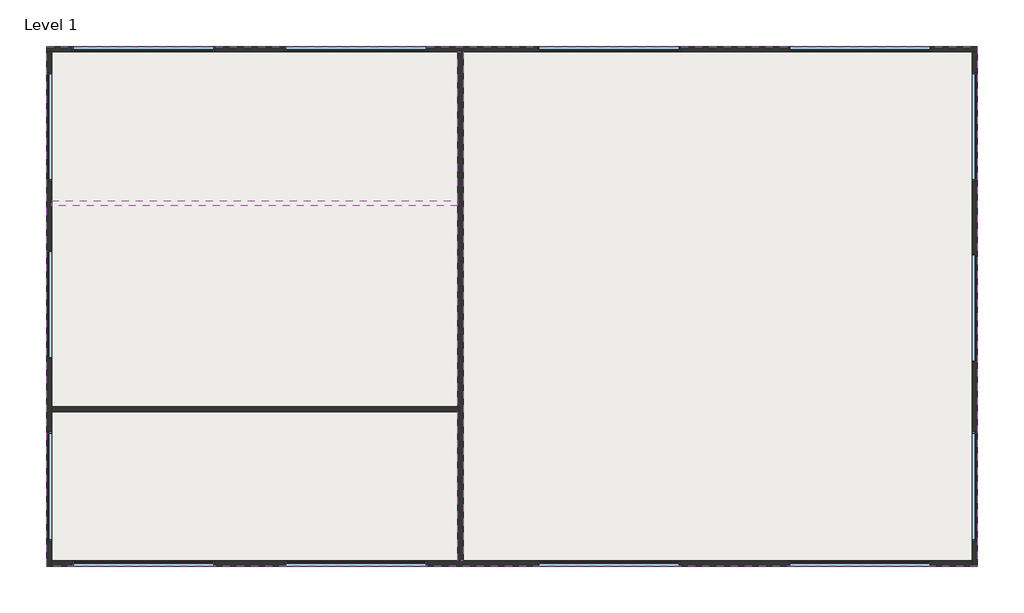
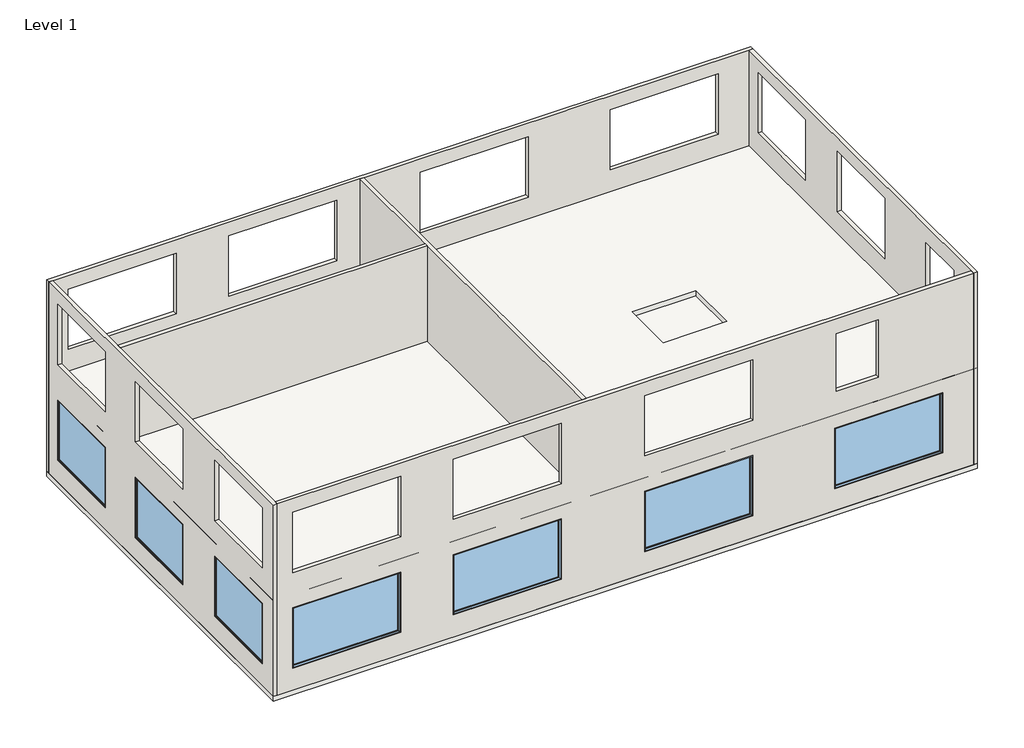
# One storey: 14 windows, 8 walls, 2 slabs.
"""IFC4 building model written with IfcOpenShell, lengths in millimetres."""

import ifcopenshell
import ifcopenshell.guid

model = None  # the IFC model being written
_history = None  # IfcOwnerHistory: only IFC2X3 demands one
_inside = {}  # id of a spatial element -> (the spatial element, [elements in it])
_under = {}  # id of a project, library or spatial element -> (it, [spatial elements below it])
_declared = {}  # id of a project -> (the project, [libraries it declares])
_typed = {}  # id of a type object -> (the type object, [elements of that type])
_made_of = {}  # id of a material, layer set ... -> (it, [elements and type objects made of it])


def new_model(schema):
    """Start an empty IFC model of exactly this schema.

    Asked for "IFC4X3", IfcOpenShell would pick the latest addendum, in which some entities
    have other attributes; the version numbers below select the first issue.
    IFC2X3 requires an IfcOwnerHistory on every rooted entity: one is made here for all.
    """
    global model, _history
    if schema == "IFC4X3":
        model = ifcopenshell.file(schema_version=(4, 3, 0, 0))
    else:
        model = ifcopenshell.file(schema=schema)
    _inside.clear()
    _under.clear()
    _declared.clear()
    _typed.clear()
    _made_of.clear()
    _history = None
    if model.schema == "IFC2X3":
        org = make("IfcOrganization", Name="unknown")
        user = make(
            "IfcPersonAndOrganization",
            ThePerson=make("IfcPerson", FamilyName="unknown"),
            TheOrganization=org,
        )
        app = make(
            "IfcApplication",
            ApplicationDeveloper=org,
            Version="unknown",
            ApplicationFullName="unknown",
            ApplicationIdentifier="unknown",
        )
        _history = make(
            "IfcOwnerHistory",
            OwningUser=user,
            OwningApplication=app,
            ChangeAction="ADDED",
            CreationDate=0,
        )
    return model


def make(cls, **values):
    """One entity of the class cls with the attributes given. An attribute that is None is left unset."""
    return model.create_entity(
        cls, **{name: value for name, value in values.items() if value is not None}
    )


def rooted(cls, **values):
    """An entity with a GlobalId (a new one), such as an element, a storey or a relation."""
    return make(cls, GlobalId=ifcopenshell.guid.new(), OwnerHistory=_history, **values)


def si_unit(unit_type, name, prefix=None):
    """IfcSIUnit, for example si_unit("LENGTHUNIT", "METRE", prefix="MILLI")."""
    return make("IfcSIUnit", UnitType=unit_type, Prefix=prefix, Name=name)


def assignment(units):
    """IfcUnitAssignment: the units of a project."""
    return None if units is None else make("IfcUnitAssignment", Units=units)


def point(xyz):
    """IfcCartesianPoint."""
    return None if xyz is None else make("IfcCartesianPoint", Coordinates=xyz)


def direction(xyz):
    """IfcDirection."""
    return None if xyz is None else make("IfcDirection", DirectionRatios=xyz)


def frame(location, z_axis=None, x_axis=None):
    """IfcAxis2Placement3D, a coordinate frame: its origin and axes. An axis left out is left unset."""
    return make(
        "IfcAxis2Placement3D",
        Location=point(location),
        Axis=direction(z_axis),
        RefDirection=direction(x_axis),
    )


def origin():
    """The frame at (0, 0, 0) with its axes left unset."""
    return frame((0.0, 0.0, 0.0))


def origin_with_axes():
    """The frame at (0, 0, 0) with the z axis (0, 0, 1) and the x axis (1, 0, 0) written out."""
    return frame((0.0, 0.0, 0.0), z_axis=(0.0, 0.0, 1.0), x_axis=(1.0, 0.0, 0.0))


def place(relative_to, where):
    """IfcLocalPlacement: puts the frame where relative to a parent placement (None: the world)."""
    return make(
        "IfcLocalPlacement", PlacementRelTo=relative_to, RelativePlacement=where
    )


def context(
    kind, dimensions, precision=None, world=None, true_north=None, identifier=None
):
    """IfcGeometricRepresentationContext, for example the 3D "Model" context."""
    return make(
        "IfcGeometricRepresentationContext",
        ContextIdentifier=identifier,
        ContextType=kind,
        CoordinateSpaceDimension=dimensions,
        Precision=precision,
        WorldCoordinateSystem=world,
        TrueNorth=true_north,
    )


def project(units=None, contexts=None):
    """IfcProject with its units and contexts."""
    return rooted(
        "IfcProject",
        Name="project",
        RepresentationContexts=contexts,
        UnitsInContext=assignment(units),
    )


def spatial(cls, under=None, at=None, **own):
    """A site, building, storey or space (cls), placed at a placement, below another one or the project."""
    s = rooted(cls, ObjectPlacement=at, **own)
    if under is not None:
        _under.setdefault(under.id(), (under, []))[1].append(s)
    return s


def polyline(points):
    """IfcPolyline through the points."""
    return make("IfcPolyline", Points=[point(p) for p in points])


def outline(outer, holes=None, kind="AREA"):
    """IfcArbitraryClosedProfileDef: a profile drawn as a closed curve; with holes, ...WithVoids."""
    if holes is None:
        return make("IfcArbitraryClosedProfileDef", ProfileType=kind, OuterCurve=outer)
    return make(
        "IfcArbitraryProfileDefWithVoids",
        ProfileType=kind,
        OuterCurve=outer,
        InnerCurves=holes,
    )


def extrude(swept, where, along, depth):
    """IfcExtrudedAreaSolid: the profile swept, set in the frame where, extruded along a direction by depth."""
    return make(
        "IfcExtrudedAreaSolid",
        SweptArea=swept,
        Position=where,
        ExtrudedDirection=direction(along),
        Depth=depth,
    )


def faces_of(points, faces, orient=None, outer=None):
    """IfcFace entities. A face is a list of loops; a loop is a list of indices into points, from 0.

    orient and outer hold one flag for each loop. By default every Orientation is true, the
    first loop of a face is its IfcFaceOuterBound and the others are IfcFaceBound.
    """
    made = []
    for i, loops in enumerate(faces):
        bounds = []
        for j, loop in enumerate(loops):
            is_outer = j == 0 if outer is None else outer[i][j]
            bounds.append(
                make(
                    "IfcFaceOuterBound" if is_outer else "IfcFaceBound",
                    Bound=make("IfcPolyLoop", Polygon=[points[k] for k in loop]),
                    Orientation=True if orient is None else orient[i][j],
                )
            )
        made.append(make("IfcFace", Bounds=bounds))
    return made


def faceted_brep(points, faces, orient=None, outer=None, voids=None):
    """IfcFacetedBrep: a solid bounded by flat faces; with voids (closed shells), ...WithVoids."""
    shared = [point(p) for p in points]
    hull = make("IfcClosedShell", CfsFaces=faces_of(shared, faces, orient, outer))
    if voids is None:
        return make("IfcFacetedBrep", Outer=hull)
    return make(
        "IfcFacetedBrepWithVoids",
        Outer=hull,
        Voids=[
            make(cls, CfsFaces=faces_of(shared, fs, o, b)) for cls, fs, o, b in voids
        ],
    )


def shape(context_of_items, identifier, shape_type, items):
    """IfcShapeRepresentation: the items that make up one representation, for example the "Body"."""
    return make(
        "IfcShapeRepresentation",
        ContextOfItems=context_of_items,
        RepresentationIdentifier=identifier,
        RepresentationType=shape_type,
        Items=items,
    )


def source(mapping_origin, context_of_items, identifier, shape_type, items):
    """IfcRepresentationMap: a shape defined once, which mapped items show again and again."""
    return make(
        "IfcRepresentationMap",
        MappingOrigin=mapping_origin,
        MappedRepresentation=shape(context_of_items, identifier, shape_type, items),
    )


def transform(
    local_origin,
    x_axis=None,
    y_axis=None,
    z_axis=None,
    scale=None,
    scale2=None,
    scale3=None,
    uniform=True,
):
    """IfcCartesianTransformationOperator3D, or its non-uniform kind. x_axis, y_axis, z_axis: its Axis1, 2, 3."""
    if uniform:
        return make(
            "IfcCartesianTransformationOperator3D",
            Axis1=direction(x_axis),
            Axis2=direction(y_axis),
            LocalOrigin=point(local_origin),
            Scale=scale,
            Axis3=direction(z_axis),
        )
    return make(
        "IfcCartesianTransformationOperator3DnonUniform",
        Axis1=direction(x_axis),
        Axis2=direction(y_axis),
        LocalOrigin=point(local_origin),
        Scale=scale,
        Axis3=direction(z_axis),
        Scale2=scale2,
        Scale3=scale3,
    )


def mapped(mapping_source, mapping_target):
    """IfcMappedItem: shows the shape of a source again, moved by a transform."""
    return make(
        "IfcMappedItem", MappingSource=mapping_source, MappingTarget=mapping_target
    )


def made_of(thing, what):
    """Note that an element or type object is made of a material, layer set ...; save() writes the relation."""
    if what is not None:
        _made_of.setdefault(what.id(), (what, []))[1].append(thing)
    return thing


def element(
    cls,
    number,
    at=None,
    inside=None,
    cuts=None,
    type_object=None,
    material=None,
    context=None,
    identifier="Body",
    shape_type=None,
    held_by="IfcProductDefinitionShape",
    body=None,
    shapes=None,
    **own,
):
    """One element of the class cls, such as IfcWall. Its Tag is "e" and its number.

    at: its placement. inside: the storey or other place that contains it. cuts: it is an
    opening in that element (IfcRelVoidsElement). A single representation is given by context,
    identifier, shape_type and body (its items); several are given by shapes. held_by: the class
    of the entity that holds the representations. save() writes the other relations.
    """
    e = rooted(cls, Tag="e%d" % number, ObjectPlacement=at, **own)
    if body is not None:
        shapes = [shape(context, identifier, shape_type, body)]
    if shapes is not None:
        e.Representation = make(held_by, Representations=shapes)
    if inside is not None:
        _inside.setdefault(inside.id(), (inside, []))[1].append(e)
    if cuts is not None:
        rooted(
            "IfcRelVoidsElement", RelatingBuildingElement=cuts, RelatedOpeningElement=e
        )
    if type_object is not None:
        _typed.setdefault(type_object.id(), (type_object, []))[1].append(e)
    return made_of(e, material)


def aggregate(whole, parts):
    """IfcRelAggregates: a whole, such as a stair, and the parts it consists of."""
    return rooted("IfcRelAggregates", RelatingObject=whole, RelatedObjects=parts)


def save(model, path):
    """Write the relations noted so far, then the file.

    IfcRelAggregates (storeys below a building ...), IfcRelContainedInSpatialStructure (elements
    in a storey), IfcRelDefinesByType, IfcRelAssociatesMaterial and IfcRelDeclares: one each for
    every whole, place, type object, material and project.
    """
    for whole, parts in _under.values():
        aggregate(whole, parts)
    for where, things in _inside.values():
        rooted(
            "IfcRelContainedInSpatialStructure",
            RelatedElements=things,
            RelatingStructure=where,
        )
    for kind, things in _typed.values():
        rooted("IfcRelDefinesByType", RelatedObjects=things, RelatingType=kind)
    for what, things in _made_of.values():
        rooted("IfcRelAssociatesMaterial", RelatedObjects=things, RelatingMaterial=what)
    for by, libraries in _declared.values():
        rooted("IfcRelDeclares", RelatingContext=by, RelatedDefinitions=libraries)
    model.write(path)


def m_fixed_2500x_4228mm_fd5e51e7(model_context):
    return source(origin(), model_context, "Body", "SweptSolid", [
        extrude(outline(polyline([(-2050.8, 54.2), (2050.8, 54.2), (2050.8, 42.2), (-2050.8, 42.2), (-2050.8, 54.2)])), frame((0.0, 0.0, 368.0), z_axis=(0.0, 0.0, 1.0), x_axis=(1.0, 0.0, 0.0)), (0.0, 0.0, 1.0), 2374.0),
        extrude(outline(polyline([(2786.0, -2094.8), (324.0, -2094.8), (324.0, 2094.8), (2786.0, 2094.8), (2786.0, -2094.8)]), holes=[polyline([(2742.0, -2050.8), (2742.0, 2050.8), (368.0, 2050.8), (368.0, -2050.8), (2742.0, -2050.8)])]), frame((0.0, 26.2, 0.0), z_axis=(0.0, 1.0, 0.0), x_axis=(0.0, 0.0, 1.0)), (0.0, 0.0, 1.0), 44.0),
        extrude(outline(polyline([(2805.0, -2113.8), (305.0, -2113.8), (305.0, 2113.8), (2805.0, 2113.8), (2805.0, -2113.8)]), holes=[polyline([(2786.0, -2094.8), (2786.0, 2094.8), (324.0, 2094.8), (324.0, -2094.8), (2786.0, -2094.8)])]), frame((0.0, 26.2, 0.0), z_axis=(0.0, 1.0, 0.0), x_axis=(0.0, 0.0, 1.0)), (0.0, 0.0, 1.0), 63.0),
        extrude(outline(polyline([(2805.0, -2113.8), (305.0, -2113.8), (305.0, 2113.8), (2805.0, 2113.8), (2805.0, -2113.8)]), holes=[polyline([(2773.0, -2081.8), (2773.0, 2081.8), (337.0, 2081.8), (337.0, -2081.8), (2773.0, -2081.8)])]), frame((0.0, -63.2, 0.0), z_axis=(0.0, 1.0, 0.0), x_axis=(0.0, 0.0, 1.0)), (0.0, 0.0, 1.0), 89.4),
    ])


def m_fixed_2500x_4228mm_f14c179f(model_context):
    return source(origin(), model_context, "Body", "SweptSolid", [
        extrude(outline(polyline([(-2050.8, -54.2), (-2050.8, -42.2), (2050.8, -42.2), (2050.8, -54.2), (-2050.8, -54.2)])), frame((0.0, 0.0, 368.0), z_axis=(0.0, 0.0, 1.0), x_axis=(1.0, 0.0, 0.0)), (0.0, 0.0, 1.0), 2374.0),
        extrude(outline(polyline([(2786.0, -2094.8), (324.0, -2094.8), (324.0, 2094.8), (2786.0, 2094.8), (2786.0, -2094.8)]), holes=[polyline([(2742.0, -2050.8), (2742.0, 2050.8), (368.0, 2050.8), (368.0, -2050.8), (2742.0, -2050.8)])]), frame((0.0, -70.2, 0.0), z_axis=(0.0, 1.0, 0.0), x_axis=(0.0, 0.0, 1.0)), (0.0, 0.0, 1.0), 44.0),
        extrude(outline(polyline([(2805.0, -2113.8), (305.0, -2113.8), (305.0, 2113.8), (2805.0, 2113.8), (2805.0, -2113.8)]), holes=[polyline([(2786.0, -2094.8), (2786.0, 2094.8), (324.0, 2094.8), (324.0, -2094.8), (2786.0, -2094.8)])]), frame((0.0, -89.2, 0.0), z_axis=(0.0, 1.0, 0.0), x_axis=(0.0, 0.0, 1.0)), (0.0, 0.0, 1.0), 63.0),
        extrude(outline(polyline([(2805.0, -2113.8), (305.0, -2113.8), (305.0, 2113.8), (2805.0, 2113.8), (2805.0, -2113.8)]), holes=[polyline([(2773.0, -2081.8), (2773.0, 2081.8), (337.0, 2081.8), (337.0, -2081.8), (2773.0, -2081.8)])]), frame((0.0, -26.2, 0.0), z_axis=(0.0, 1.0, 0.0), x_axis=(0.0, 0.0, 1.0)), (0.0, 0.0, 1.0), 89.4),
    ])


def m_fixed_2500x_3220mm_df94f4d0(model_context):
    return source(origin(), model_context, "Body", "SweptSolid", [
        extrude(outline(polyline([(-1546.8, 54.2), (1546.8, 54.2), (1546.8, 42.2), (-1546.8, 42.2), (-1546.8, 54.2)])), frame((0.0, 0.0, 368.0), z_axis=(0.0, 0.0, 1.0), x_axis=(1.0, 0.0, 0.0)), (0.0, 0.0, 1.0), 2374.0),
        extrude(outline(polyline([(2786.0, -1590.8), (324.0, -1590.8), (324.0, 1590.8), (2786.0, 1590.8), (2786.0, -1590.8)]), holes=[polyline([(2742.0, -1546.8), (2742.0, 1546.8), (368.0, 1546.8), (368.0, -1546.8), (2742.0, -1546.8)])]), frame((0.0, 26.2, 0.0), z_axis=(0.0, 1.0, 0.0), x_axis=(0.0, 0.0, 1.0)), (0.0, 0.0, 1.0), 44.0),
        extrude(outline(polyline([(2805.0, -1609.8), (305.0, -1609.8), (305.0, 1609.8), (2805.0, 1609.8), (2805.0, -1609.8)]), holes=[polyline([(2786.0, -1590.8), (2786.0, 1590.8), (324.0, 1590.8), (324.0, -1590.8), (2786.0, -1590.8)])]), frame((0.0, 26.2, 0.0), z_axis=(0.0, 1.0, 0.0), x_axis=(0.0, 0.0, 1.0)), (0.0, 0.0, 1.0), 63.0),
        extrude(outline(polyline([(2805.0, -1609.8), (305.0, -1609.8), (305.0, 1609.8), (2805.0, 1609.8), (2805.0, -1609.8)]), holes=[polyline([(2773.0, -1577.8), (2773.0, 1577.8), (337.0, 1577.8), (337.0, -1577.8), (2773.0, -1577.8)])]), frame((0.0, -63.2, 0.0), z_axis=(0.0, 1.0, 0.0), x_axis=(0.0, 0.0, 1.0)), (0.0, 0.0, 1.0), 89.4),
    ])


def m_fixed_2500x_3220mm_8b997f8c(model_context):
    return source(origin(), model_context, "Body", "SweptSolid", [
        extrude(outline(polyline([(-1546.8, -54.2), (-1546.8, -42.2), (1546.8, -42.2), (1546.8, -54.2), (-1546.8, -54.2)])), frame((0.0, 0.0, 368.0), z_axis=(0.0, 0.0, 1.0), x_axis=(1.0, 0.0, 0.0)), (0.0, 0.0, 1.0), 2374.0),
        extrude(outline(polyline([(2786.0, -1590.8), (324.0, -1590.8), (324.0, 1590.8), (2786.0, 1590.8), (2786.0, -1590.8)]), holes=[polyline([(2742.0, -1546.8), (2742.0, 1546.8), (368.0, 1546.8), (368.0, -1546.8), (2742.0, -1546.8)])]), frame((0.0, -70.2, 0.0), z_axis=(0.0, 1.0, 0.0), x_axis=(0.0, 0.0, 1.0)), (0.0, 0.0, 1.0), 44.0),
        extrude(outline(polyline([(2805.0, -1609.8), (305.0, -1609.8), (305.0, 1609.8), (2805.0, 1609.8), (2805.0, -1609.8)]), holes=[polyline([(2786.0, -1590.8), (2786.0, 1590.8), (324.0, 1590.8), (324.0, -1590.8), (2786.0, -1590.8)])]), frame((0.0, -89.2, 0.0), z_axis=(0.0, 1.0, 0.0), x_axis=(0.0, 0.0, 1.0)), (0.0, 0.0, 1.0), 63.0),
        extrude(outline(polyline([(2805.0, -1609.8), (305.0, -1609.8), (305.0, 1609.8), (2805.0, 1609.8), (2805.0, -1609.8)]), holes=[polyline([(2773.0, -1577.8), (2773.0, 1577.8), (337.0, 1577.8), (337.0, -1577.8), (2773.0, -1577.8)])]), frame((0.0, -26.2, 0.0), z_axis=(0.0, 1.0, 0.0), x_axis=(0.0, 0.0, 1.0)), (0.0, 0.0, 1.0), 89.4),
    ])


model = new_model("IFC4")

# Units and contexts
model_context = context("Model", 3, world=origin())
ifc_project = project(units=[si_unit("LENGTHUNIT", "METRE", prefix="MILLI")], contexts=[model_context])

# Site, building, storey
site = spatial("IfcSite", under=ifc_project)
building = spatial("IfcBuilding", under=site)
storey = spatial("IfcBuildingStorey", under=building, Name="Level 1", Elevation=0.0)

# Slabs
placement = place(None, origin())
element("IfcSlab", 1, ObjectType="160mm Concrete With 50mm Metal Deck", at=placement, inside=storey, context=model_context, shape_type="Brep", body=[
    faceted_brep([(29068.464681, 11296.9802217, -210.0), (29068.464681, -4095.4197783, -210.0), (1484.064681, -4095.4197783, -210.0), (1484.064681, 11296.9802217, -210.0), (29068.464681, 11296.9802217, 0.0), (1484.064681, 11296.9802217, 0.0), (1484.064681, 11144.5802217, 0.0), (1484.064681, -4095.4197783, 0.0), (28916.064681, -4095.4197783, 0.0), (29068.464681, -4095.4197783, 0.0), (29068.464681, 11144.5802217, 0.0)], [[[0, 1, 2, 3]], [[4, 5, 6, 7, 8, 9, 10]], [[1, 0, 4, 10, 9]], [[2, 1, 9, 8, 7]], [[3, 2, 7, 6, 5]], [[0, 3, 5, 4]]]),
])
element("IfcSlab", 2, ObjectType="160mm Concrete With 50mm Metal Deck", at=placement, inside=storey, context=model_context, shape_type="SweptSolid", body=[
    extrude(outline(polyline([(29068.464681, 11296.9802217), (29068.464681, -4095.4197783), (1484.064681, -4095.4197783), (1484.064681, 11296.9802217), (29068.464681, 11296.9802217)]), holes=[polyline([(23070.5967133, 4620.1802217), (20570.5967133, 4620.1802217), (20570.5967133, 2520.1802217), (23070.5967133, 2520.1802217), (23070.5967133, 4620.1802217)])]), frame((0.0, 0.0, 3752.4), z_axis=(0.0, 0.0, 1.0), x_axis=(1.0, 0.0, 0.0)), (0.0, 0.0, 1.0), 210.0),
])

# Walls
element("IfcWall", 3, ObjectType="Generic - 152.4mm", at=placement, inside=storey, context=model_context, shape_type="Brep", body=[
    faceted_brep([(1484.064681, 11144.5802217, 0.0), (1636.464681, 11144.5802217, 0.0), (13676.064681, 11144.5802217, 0.0), (13828.464681, 11144.5802217, 0.0), (28916.064681, 11144.5802217, 0.0), (29068.464681, 11144.5802217, 0.0), (29068.464681, 11144.5802217, 7924.8), (28916.064681, 11144.5802217, 7924.8), (23222.9967133, 11144.5802217, 7924.8), (23070.5967133, 11144.5802217, 7924.8), (20570.5967133, 11144.5802217, 7924.8), (20418.1967133, 11144.5802217, 7924.8), (13828.464681, 11144.5802217, 7924.8), (13676.064681, 11144.5802217, 7924.8), (1636.464681, 11144.5802217, 7924.8), (1484.064681, 11144.5802217, 7924.8), (6474.064681, 11144.5802217, 902.4), (2246.464681, 11144.5802217, 902.4), (2246.464681, 11144.5802217, 3402.4), (6474.064681, 11144.5802217, 3402.4), (12766.064681, 11144.5802217, 902.4), (8538.464681, 11144.5802217, 902.4), (8538.464681, 11144.5802217, 3402.4), (12766.064681, 11144.5802217, 3402.4), (20266.064681, 11144.5802217, 902.4), (16038.464681, 11144.5802217, 902.4), (16038.464681, 11144.5802217, 3402.4), (20266.064681, 11144.5802217, 3402.4), (27706.064681, 11144.5802217, 902.4), (23478.464681, 11144.5802217, 902.4), (23478.464681, 11144.5802217, 3402.4), (27706.064681, 11144.5802217, 3402.4), (27706.064681, 11144.5802217, 4862.4), (23478.464681, 11144.5802217, 4862.4), (23478.464681, 11144.5802217, 7362.4), (27706.064681, 11144.5802217, 7362.4), (20266.064681, 11144.5802217, 4862.4), (16038.464681, 11144.5802217, 4862.4), (16038.464681, 11144.5802217, 7362.4), (20266.064681, 11144.5802217, 7362.4), (12766.064681, 11144.5802217, 4862.4), (8538.464681, 11144.5802217, 4862.4), (8538.464681, 11144.5802217, 7362.4), (12766.064681, 11144.5802217, 7362.4), (6474.064681, 11144.5802217, 4862.4), (2246.464681, 11144.5802217, 4862.4), (2246.464681, 11144.5802217, 7362.4), (6474.064681, 11144.5802217, 7362.4), (1484.064681, 11296.9802217, 0.0), (1484.064681, 11296.9802217, 7924.8), (29068.464681, 11296.9802217, 7924.8), (29068.464681, 11296.9802217, 0.0), (6474.064681, 11296.9802217, 902.4), (6474.064681, 11296.9802217, 3402.4), (2246.464681, 11296.9802217, 3402.4), (2246.464681, 11296.9802217, 902.4), (12766.064681, 11296.9802217, 902.4), (12766.064681, 11296.9802217, 3402.4), (8538.464681, 11296.9802217, 3402.4), (8538.464681, 11296.9802217, 902.4), (20266.064681, 11296.9802217, 902.4), (20266.064681, 11296.9802217, 3402.4), (16038.464681, 11296.9802217, 3402.4), (16038.464681, 11296.9802217, 902.4), (27706.064681, 11296.9802217, 902.4), (27706.064681, 11296.9802217, 3402.4), (23478.464681, 11296.9802217, 3402.4), (23478.464681, 11296.9802217, 902.4), (27706.064681, 11296.9802217, 4862.4), (27706.064681, 11296.9802217, 7362.4), (23478.464681, 11296.9802217, 7362.4), (23478.464681, 11296.9802217, 4862.4), (20266.064681, 11296.9802217, 4862.4), (20266.064681, 11296.9802217, 7362.4), (16038.464681, 11296.9802217, 7362.4), (16038.464681, 11296.9802217, 4862.4), (12766.064681, 11296.9802217, 4862.4), (12766.064681, 11296.9802217, 7362.4), (8538.464681, 11296.9802217, 7362.4), (8538.464681, 11296.9802217, 4862.4), (6474.064681, 11296.9802217, 4862.4), (6474.064681, 11296.9802217, 7362.4), (2246.464681, 11296.9802217, 7362.4), (2246.464681, 11296.9802217, 4862.4)], [[[0, 1, 2, 3, 4, 5, 6, 7, 8, 9, 10, 11, 12, 13, 14, 15], [16, 17, 18, 19], [20, 21, 22, 23], [24, 25, 26, 27], [28, 29, 30, 31], [32, 33, 34, 35], [36, 37, 38, 39], [40, 41, 42, 43], [44, 45, 46, 47]], [[48, 49, 50, 51], [52, 53, 54, 55], [56, 57, 58, 59], [60, 61, 62, 63], [64, 65, 66, 67], [68, 69, 70, 71], [72, 73, 74, 75], [76, 77, 78, 79], [80, 81, 82, 83]], [[5, 4, 3, 2, 1, 0, 48, 51]], [[15, 14, 13, 12, 11, 10, 9, 8, 7, 6, 50, 49]], [[6, 5, 51, 50]], [[0, 15, 49, 48]], [[53, 52, 16, 19]], [[54, 53, 19, 18]], [[55, 54, 18, 17]], [[52, 55, 17, 16]], [[57, 56, 20, 23]], [[58, 57, 23, 22]], [[59, 58, 22, 21]], [[56, 59, 21, 20]], [[61, 60, 24, 27]], [[62, 61, 27, 26]], [[63, 62, 26, 25]], [[60, 63, 25, 24]], [[65, 64, 28, 31]], [[66, 65, 31, 30]], [[67, 66, 30, 29]], [[64, 67, 29, 28]], [[69, 68, 32, 35]], [[70, 69, 35, 34]], [[71, 70, 34, 33]], [[68, 71, 33, 32]], [[73, 72, 36, 39]], [[74, 73, 39, 38]], [[75, 74, 38, 37]], [[72, 75, 37, 36]], [[77, 76, 40, 43]], [[78, 77, 43, 42]], [[79, 78, 42, 41]], [[76, 79, 41, 40]], [[81, 80, 44, 47]], [[82, 81, 47, 46]], [[83, 82, 46, 45]], [[80, 83, 45, 44]]]),
])
element("IfcWall", 4, ObjectType="Generic - 152.4mm", at=placement, inside=storey, context=model_context, shape_type="Brep", body=[
    faceted_brep([(28916.064681, 11144.5802217, 0.0), (28916.064681, -3943.0197783, 0.0), (28916.064681, -4095.4197783, 0.0), (28916.064681, -4095.4197783, 7924.8), (28916.064681, -3943.0197783, 7924.8), (28916.064681, 11144.5802217, 7924.8), (28916.064681, -3343.0197783, 902.4), (28916.064681, -123.4197783, 902.4), (28916.064681, -123.4197783, 3402.4), (28916.064681, -3343.0197783, 3402.4), (28916.064681, 1942.9802217, 902.4), (28916.064681, 5162.5802217, 902.4), (28916.064681, 5162.5802217, 3402.4), (28916.064681, 1942.9802217, 3402.4), (28916.064681, 7310.9802217, 902.4), (28916.064681, 10530.5802217, 902.4), (28916.064681, 10530.5802217, 3402.4), (28916.064681, 7310.9802217, 3402.4), (28916.064681, 1942.9802217, 4864.8), (28916.064681, 5162.5802217, 4864.8), (28916.064681, 5162.5802217, 7364.8), (28916.064681, 1942.9802217, 7364.8), (28916.064681, 7310.9802217, 4864.8), (28916.064681, 10530.5802217, 4864.8), (28916.064681, 10530.5802217, 7364.8), (28916.064681, 7310.9802217, 7364.8), (28916.064681, -853.3553952, 7228.0785572), (28916.064681, -2753.3553952, 7228.0785572), (28916.064681, -2753.3553952, 4828.0785572), (28916.064681, -853.3553952, 4828.0785572), (29068.464681, 11144.5802217, 0.0), (29068.464681, 11144.5802217, 7924.8), (29068.464681, -4095.4197783, 7924.8), (29068.464681, -4095.4197783, 0.0), (29068.464681, -3343.0197783, 902.4), (29068.464681, -3343.0197783, 3402.4), (29068.464681, -123.4197783, 3402.4), (29068.464681, -123.4197783, 902.4), (29068.464681, 1942.9802217, 902.4), (29068.464681, 1942.9802217, 3402.4), (29068.464681, 5162.5802217, 3402.4), (29068.464681, 5162.5802217, 902.4), (29068.464681, 7310.9802217, 902.4), (29068.464681, 7310.9802217, 3402.4), (29068.464681, 10530.5802217, 3402.4), (29068.464681, 10530.5802217, 902.4), (29068.464681, 1942.9802217, 4864.8), (29068.464681, 1942.9802217, 7364.8), (29068.464681, 5162.5802217, 7364.8), (29068.464681, 5162.5802217, 4864.8), (29068.464681, 7310.9802217, 4864.8), (29068.464681, 7310.9802217, 7364.8), (29068.464681, 10530.5802217, 7364.8), (29068.464681, 10530.5802217, 4864.8), (29068.464681, -853.3553952, 7228.0785572), (29068.464681, -853.3553952, 4828.0785572), (29068.464681, -2753.3553952, 4828.0785572), (29068.464681, -2753.3553952, 7228.0785572)], [[[0, 1, 2, 3, 4, 5], [6, 7, 8, 9], [10, 11, 12, 13], [14, 15, 16, 17], [18, 19, 20, 21], [22, 23, 24, 25], [26, 27, 28, 29]], [[30, 31, 32, 33], [34, 35, 36, 37], [38, 39, 40, 41], [42, 43, 44, 45], [46, 47, 48, 49], [50, 51, 52, 53], [54, 55, 56, 57]], [[0, 5, 31, 30]], [[35, 34, 6, 9]], [[36, 35, 9, 8]], [[37, 36, 8, 7]], [[34, 37, 7, 6]], [[39, 38, 10, 13]], [[40, 39, 13, 12]], [[41, 40, 12, 11]], [[38, 41, 11, 10]], [[43, 42, 14, 17]], [[44, 43, 17, 16]], [[45, 44, 16, 15]], [[42, 45, 15, 14]], [[3, 2, 33, 32]], [[47, 46, 18, 21]], [[48, 47, 21, 20]], [[49, 48, 20, 19]], [[46, 49, 19, 18]], [[51, 50, 22, 25]], [[52, 51, 25, 24]], [[53, 52, 24, 23]], [[50, 53, 23, 22]], [[2, 1, 0, 30, 33]], [[5, 4, 3, 32, 31]], [[27, 26, 54, 57]], [[28, 27, 57, 56]], [[29, 28, 56, 55]], [[26, 29, 55, 54]]]),
])
element("IfcWall", 5, ObjectType="Generic - 152.4mm", at=placement, inside=storey, context=model_context, shape_type="Brep", body=[
    faceted_brep([(28916.064681, -3943.0197783, 0.0), (13828.464681, -3943.0197783, 0.0), (13676.064681, -3943.0197783, 0.0), (1636.464681, -3943.0197783, 0.0), (1636.464681, -3943.0197783, 7924.8), (13676.064681, -3943.0197783, 7924.8), (13828.464681, -3943.0197783, 7924.8), (20418.1967133, -3943.0197783, 7924.8), (20570.5967133, -3943.0197783, 7924.8), (23070.5967133, -3943.0197783, 7924.8), (23222.9967133, -3943.0197783, 7924.8), (28916.064681, -3943.0197783, 7924.8), (27706.064681, -3943.0197783, 902.4), (27706.064681, -3943.0197783, 3402.4), (23478.464681, -3943.0197783, 3402.4), (23478.464681, -3943.0197783, 902.4), (20266.064681, -3943.0197783, 902.4), (20266.064681, -3943.0197783, 3402.4), (16038.464681, -3943.0197783, 3402.4), (16038.464681, -3943.0197783, 902.4), (12766.064681, -3943.0197783, 902.4), (12766.064681, -3943.0197783, 3402.4), (8538.464681, -3943.0197783, 3402.4), (8538.464681, -3943.0197783, 902.4), (6474.064681, -3943.0197783, 902.4), (6474.064681, -3943.0197783, 3402.4), (2246.464681, -3943.0197783, 3402.4), (2246.464681, -3943.0197783, 902.4), (20266.064681, -3943.0197783, 4862.4), (20266.064681, -3943.0197783, 7362.4), (16038.464681, -3943.0197783, 7362.4), (16038.464681, -3943.0197783, 4862.4), (12766.064681, -3943.0197783, 4862.4), (12766.064681, -3943.0197783, 7362.4), (8538.464681, -3943.0197783, 7362.4), (8538.464681, -3943.0197783, 4862.4), (6474.064681, -3943.0197783, 4862.4), (6474.064681, -3943.0197783, 7362.4), (2246.464681, -3943.0197783, 7362.4), (2246.464681, -3943.0197783, 4862.4), (25185.6307376, -3943.0197783, 7299.4), (23541.464681, -3943.0197783, 7299.4), (23541.464681, -3943.0197783, 4925.4), (25185.6307376, -3943.0197783, 4925.4), (28916.064681, -4095.4197783, 0.0), (28916.064681, -4095.4197783, 7924.8), (1636.464681, -4095.4197783, 7924.8), (1636.464681, -4095.4197783, 0.0), (27706.064681, -4095.4197783, 902.4), (23478.464681, -4095.4197783, 902.4), (23478.464681, -4095.4197783, 3402.4), (27706.064681, -4095.4197783, 3402.4), (20266.064681, -4095.4197783, 902.4), (16038.464681, -4095.4197783, 902.4), (16038.464681, -4095.4197783, 3402.4), (20266.064681, -4095.4197783, 3402.4), (12766.064681, -4095.4197783, 902.4), (8538.464681, -4095.4197783, 902.4), (8538.464681, -4095.4197783, 3402.4), (12766.064681, -4095.4197783, 3402.4), (6474.064681, -4095.4197783, 902.4), (2246.464681, -4095.4197783, 902.4), (2246.464681, -4095.4197783, 3402.4), (6474.064681, -4095.4197783, 3402.4), (20266.064681, -4095.4197783, 4862.4), (16038.464681, -4095.4197783, 4862.4), (16038.464681, -4095.4197783, 7362.4), (20266.064681, -4095.4197783, 7362.4), (12766.064681, -4095.4197783, 4862.4), (8538.464681, -4095.4197783, 4862.4), (8538.464681, -4095.4197783, 7362.4), (12766.064681, -4095.4197783, 7362.4), (6474.064681, -4095.4197783, 4862.4), (2246.464681, -4095.4197783, 4862.4), (2246.464681, -4095.4197783, 7362.4), (6474.064681, -4095.4197783, 7362.4), (25185.6307376, -4095.4197783, 7299.4), (25185.6307376, -4095.4197783, 4925.4), (23541.464681, -4095.4197783, 4925.4), (23541.464681, -4095.4197783, 7299.4)], [[[0, 1, 2, 3, 4, 5, 6, 7, 8, 9, 10, 11], [12, 13, 14, 15], [16, 17, 18, 19], [20, 21, 22, 23], [24, 25, 26, 27], [28, 29, 30, 31], [32, 33, 34, 35], [36, 37, 38, 39], [40, 41, 42, 43]], [[44, 45, 46, 47], [48, 49, 50, 51], [52, 53, 54, 55], [56, 57, 58, 59], [60, 61, 62, 63], [64, 65, 66, 67], [68, 69, 70, 71], [72, 73, 74, 75], [76, 77, 78, 79]], [[13, 12, 48, 51]], [[14, 13, 51, 50]], [[15, 14, 50, 49]], [[12, 15, 49, 48]], [[17, 16, 52, 55]], [[18, 17, 55, 54]], [[19, 18, 54, 53]], [[16, 19, 53, 52]], [[21, 20, 56, 59]], [[22, 21, 59, 58]], [[23, 22, 58, 57]], [[20, 23, 57, 56]], [[25, 24, 60, 63]], [[26, 25, 63, 62]], [[27, 26, 62, 61]], [[24, 27, 61, 60]], [[0, 11, 45, 44]], [[4, 3, 47, 46]], [[29, 28, 64, 67]], [[30, 29, 67, 66]], [[31, 30, 66, 65]], [[28, 31, 65, 64]], [[33, 32, 68, 71]], [[34, 33, 71, 70]], [[35, 34, 70, 69]], [[32, 35, 69, 68]], [[37, 36, 72, 75]], [[38, 37, 75, 74]], [[39, 38, 74, 73]], [[36, 39, 73, 72]], [[3, 2, 1, 0, 44, 47]], [[11, 10, 9, 8, 7, 6, 5, 4, 46, 45]], [[41, 40, 76, 79]], [[42, 41, 79, 78]], [[43, 42, 78, 77]], [[40, 43, 77, 76]]]),
])
element("IfcWall", 6, ObjectType="Generic - 152.4mm", at=placement, inside=storey, context=model_context, shape_type="Brep", body=[
    faceted_brep([(1636.464681, -4095.4197783, 0.0), (1636.464681, -3943.0197783, 0.0), (1636.464681, 476.5802217, 0.0), (1636.464681, 628.9802217, 0.0), (1636.464681, 11144.5802217, 0.0), (1636.464681, 11144.5802217, 7924.8), (1636.464681, 6724.9802217, 7924.8), (1636.464681, 6572.5802217, 7924.8), (1636.464681, -3943.0197783, 7924.8), (1636.464681, -4095.4197783, 7924.8), (1636.464681, 7310.9802217, 902.4), (1636.464681, 7310.9802217, 3402.4), (1636.464681, 10530.5802217, 3402.4), (1636.464681, 10530.5802217, 902.4), (1636.464681, 2042.9802217, 902.4), (1636.464681, 2042.9802217, 3402.4), (1636.464681, 5262.5802217, 3402.4), (1636.464681, 5262.5802217, 902.4), (1636.464681, -3343.0197783, 902.4), (1636.464681, -3343.0197783, 3402.4), (1636.464681, -123.4197783, 3402.4), (1636.464681, -123.4197783, 902.4), (1636.464681, -3343.0197783, 4864.8), (1636.464681, -3343.0197783, 7364.8), (1636.464681, -123.4197783, 7364.8), (1636.464681, -123.4197783, 4864.8), (1636.464681, 2042.9802217, 4864.8), (1636.464681, 2042.9802217, 7364.8), (1636.464681, 5262.5802217, 7364.8), (1636.464681, 5262.5802217, 4864.8), (1636.464681, 7310.9802217, 4864.8), (1636.464681, 7310.9802217, 7364.8), (1636.464681, 10530.5802217, 7364.8), (1636.464681, 10530.5802217, 4864.8), (1484.064681, -4095.4197783, 0.0), (1484.064681, -4095.4197783, 7924.8), (1484.064681, 11144.5802217, 7924.8), (1484.064681, 11144.5802217, 0.0), (1484.064681, 7310.9802217, 902.4), (1484.064681, 10530.5802217, 902.4), (1484.064681, 10530.5802217, 3402.4), (1484.064681, 7310.9802217, 3402.4), (1484.064681, 2042.9802217, 902.4), (1484.064681, 5262.5802217, 902.4), (1484.064681, 5262.5802217, 3402.4), (1484.064681, 2042.9802217, 3402.4), (1484.064681, -3343.0197783, 902.4), (1484.064681, -123.4197783, 902.4), (1484.064681, -123.4197783, 3402.4), (1484.064681, -3343.0197783, 3402.4), (1484.064681, -3343.0197783, 4864.8), (1484.064681, -123.4197783, 4864.8), (1484.064681, -123.4197783, 7364.8), (1484.064681, -3343.0197783, 7364.8), (1484.064681, 2042.9802217, 4864.8), (1484.064681, 5262.5802217, 4864.8), (1484.064681, 5262.5802217, 7364.8), (1484.064681, 2042.9802217, 7364.8), (1484.064681, 7310.9802217, 4864.8), (1484.064681, 10530.5802217, 4864.8), (1484.064681, 10530.5802217, 7364.8), (1484.064681, 7310.9802217, 7364.8)], [[[0, 1, 2, 3, 4, 5, 6, 7, 8, 9], [10, 11, 12, 13], [14, 15, 16, 17], [18, 19, 20, 21], [22, 23, 24, 25], [26, 27, 28, 29], [30, 31, 32, 33]], [[34, 35, 36, 37], [38, 39, 40, 41], [42, 43, 44, 45], [46, 47, 48, 49], [50, 51, 52, 53], [54, 55, 56, 57], [58, 59, 60, 61]], [[4, 3, 2, 1, 0, 34, 37]], [[9, 8, 7, 6, 5, 36, 35]], [[5, 4, 37, 36]], [[11, 10, 38, 41]], [[12, 11, 41, 40]], [[13, 12, 40, 39]], [[10, 13, 39, 38]], [[15, 14, 42, 45]], [[16, 15, 45, 44]], [[17, 16, 44, 43]], [[14, 17, 43, 42]], [[19, 18, 46, 49]], [[20, 19, 49, 48]], [[21, 20, 48, 47]], [[18, 21, 47, 46]], [[0, 9, 35, 34]], [[23, 22, 50, 53]], [[24, 23, 53, 52]], [[25, 24, 52, 51]], [[22, 25, 51, 50]], [[27, 26, 54, 57]], [[28, 27, 57, 56]], [[29, 28, 56, 55]], [[26, 29, 55, 54]], [[31, 30, 58, 61]], [[32, 31, 61, 60]], [[33, 32, 60, 59]], [[30, 33, 59, 58]]]),
])
element("IfcWall", 7, ObjectType="Generic - 152.4mm - Interior", at=placement, inside=storey, context=model_context, shape_type="Brep", body=[
    faceted_brep([(13828.464681, -3943.0197783, 0.0), (13828.464681, 11144.5802217, 0.0), (13828.464681, 11144.5802217, 3752.4), (13828.464681, -3943.0197783, 3752.4), (13676.064681, -3943.0197783, 0.0), (13676.064681, -3943.0197783, 3752.4), (13676.064681, 476.5802217, 3752.4), (13676.064681, 628.9802217, 3752.4), (13676.064681, 11144.5802217, 3752.4), (13676.064681, 11144.5802217, 0.0), (13676.064681, 628.9802217, 0.0), (13676.064681, 476.5802217, 0.0)], [[[0, 1, 2, 3]], [[4, 5, 6, 7, 8, 9, 10, 11]], [[1, 0, 4, 11, 10, 9]], [[0, 3, 5, 4]], [[2, 1, 9, 8]], [[3, 2, 8, 7, 6, 5]]]),
])
element("IfcWall", 8, ObjectType="Generic - 152.4mm - Interior", at=placement, inside=storey, context=model_context, shape_type="SweptSolid", body=[
    extrude(outline(polyline([(1636.464681, 628.9802217), (13676.064681, 628.9802217), (13676.064681, 476.5802217), (1636.464681, 476.5802217), (1636.464681, 628.9802217)])), origin_with_axes(), (0.0, 0.0, 1.0), 3752.4),
])
element("IfcWall", 9, ObjectType="Generic - 152.4mm - Interior", at=placement, inside=storey, context=model_context, shape_type="Brep", body=[
    faceted_brep([(13676.064681, 11144.5802217, 3962.4), (13676.064681, 6724.9802217, 3962.4), (13676.064681, 6572.5802217, 3962.4), (13676.064681, -3943.0197783, 3962.4), (13676.064681, -3943.0197783, 7924.8), (13676.064681, 6572.5802217, 7924.8), (13676.064681, 6724.9802217, 7924.8), (13676.064681, 11144.5802217, 7924.8), (13828.464681, 11144.5802217, 3962.4), (13828.464681, 11144.5802217, 7924.8), (13828.464681, -3943.0197783, 7924.8), (13828.464681, -3943.0197783, 3962.4)], [[[0, 1, 2, 3, 4, 5, 6, 7]], [[8, 9, 10, 11]], [[3, 2, 1, 0, 8, 11]], [[7, 6, 5, 4, 10, 9]], [[4, 3, 11, 10]], [[0, 7, 9, 8]]]),
])
element("IfcWall", 10, ObjectType="Generic - 152.4mm - Interior", at=placement, inside=storey, context=model_context, shape_type="SweptSolid", body=[
    extrude(outline(polyline([(1636.464681, 6724.9802217), (13676.064681, 6724.9802217), (13676.064681, 6572.5802217), (1636.464681, 6572.5802217), (1636.464681, 6724.9802217)])), frame((0.0, 0.0, 3962.4), z_axis=(0.0, 0.0, 1.0), x_axis=(1.0, 0.0, 0.0)), (0.0, 0.0, 1.0), 3962.4),
])

# Windows
m_fixed_2500x_4228mm_shape = m_fixed_2500x_4228mm_fd5e51e7(model_context)
element("IfcWindow", 11, ObjectType="M_Fixed : 2500X 4228mm", at=placement, inside=storey, context=model_context, shape_type="MappedRepresentation", body=[
    mapped(m_fixed_2500x_4228mm_shape, transform((4360.264681, 11233.7802217, 597.4), x_axis=(-1.0, 0.0, 0.0), y_axis=(0.0, -1.0, 0.0), z_axis=(0.0, 0.0, 1.0))),
])
element("IfcWindow", 12, ObjectType="M_Fixed : 2500X 4228mm", at=placement, inside=storey, context=model_context, shape_type="MappedRepresentation", body=[
    mapped(m_fixed_2500x_4228mm_shape, transform((10652.264681, 11233.7802217, 597.4), x_axis=(-1.0, 0.0, 0.0), y_axis=(0.0, -1.0, 0.0), z_axis=(0.0, 0.0, 1.0))),
])
element("IfcWindow", 13, ObjectType="M_Fixed : 2500X 4228mm", at=placement, inside=storey, context=model_context, shape_type="MappedRepresentation", body=[
    mapped(m_fixed_2500x_4228mm_shape, transform((18152.264681, 11233.7802217, 597.4), x_axis=(-1.0, 0.0, 0.0), y_axis=(0.0, -1.0, 0.0), z_axis=(0.0, 0.0, 1.0))),
])
element("IfcWindow", 14, ObjectType="M_Fixed : 2500X 4228mm", at=placement, inside=storey, context=model_context, shape_type="MappedRepresentation", body=[
    mapped(m_fixed_2500x_4228mm_shape, transform((25592.264681, 11233.7802217, 597.4), x_axis=(-1.0, 0.0, 0.0), y_axis=(0.0, -1.0, 0.0), z_axis=(0.0, 0.0, 1.0))),
])
m_fixed_2500x_4228mm_2_shape = m_fixed_2500x_4228mm_f14c179f(model_context)
element("IfcWindow", 15, ObjectType="M_Fixed : 2500X 4228mm", at=placement, inside=storey, context=model_context, shape_type="MappedRepresentation", body=[
    mapped(m_fixed_2500x_4228mm_2_shape, transform((4360.264681, -4032.2197783, 597.4), x_axis=(-1.0, 0.0, 0.0), y_axis=(0.0, -1.0, 0.0), z_axis=(0.0, 0.0, 1.0))),
])
element("IfcWindow", 16, ObjectType="M_Fixed : 2500X 4228mm", at=placement, inside=storey, context=model_context, shape_type="MappedRepresentation", body=[
    mapped(m_fixed_2500x_4228mm_2_shape, transform((10652.264681, -4032.2197783, 597.4), x_axis=(-1.0, 0.0, 0.0), y_axis=(0.0, -1.0, 0.0), z_axis=(0.0, 0.0, 1.0))),
])
element("IfcWindow", 17, ObjectType="M_Fixed : 2500X 4228mm", at=placement, inside=storey, context=model_context, shape_type="MappedRepresentation", body=[
    mapped(m_fixed_2500x_4228mm_2_shape, transform((18152.264681, -4032.2197783, 597.4), x_axis=(-1.0, 0.0, 0.0), y_axis=(0.0, -1.0, 0.0), z_axis=(0.0, 0.0, 1.0))),
])
element("IfcWindow", 18, ObjectType="M_Fixed : 2500X 4228mm", at=placement, inside=storey, context=model_context, shape_type="MappedRepresentation", body=[
    mapped(m_fixed_2500x_4228mm_2_shape, transform((25592.264681, -4032.2197783, 597.4), x_axis=(-1.0, 0.0, 0.0), y_axis=(0.0, -1.0, 0.0), z_axis=(0.0, 0.0, 1.0))),
])
m_fixed_2500x_3220mm_shape = m_fixed_2500x_3220mm_df94f4d0(model_context)
element("IfcWindow", 19, ObjectType="M_Fixed : 2500x 3220mm", at=placement, inside=storey, context=model_context, shape_type="MappedRepresentation", body=[
    mapped(m_fixed_2500x_3220mm_shape, transform((1573.264681, 8920.7802217, 597.4), x_axis=(0.0, 1.0, 0.0), y_axis=(-1.0, 0.0, 0.0), z_axis=(0.0, 0.0, 1.0))),
])
element("IfcWindow", 20, ObjectType="M_Fixed : 2500x 3220mm", at=placement, inside=storey, context=model_context, shape_type="MappedRepresentation", body=[
    mapped(m_fixed_2500x_3220mm_shape, transform((1573.264681, 3652.7802217, 597.4), x_axis=(0.0, 1.0, 0.0), y_axis=(-1.0, 0.0, 0.0), z_axis=(0.0, 0.0, 1.0))),
])
element("IfcWindow", 21, ObjectType="M_Fixed : 2500x 3220mm", at=placement, inside=storey, context=model_context, shape_type="MappedRepresentation", body=[
    mapped(m_fixed_2500x_3220mm_shape, transform((1573.264681, -1733.2197783, 597.4), x_axis=(0.0, 1.0, 0.0), y_axis=(-1.0, 0.0, 0.0), z_axis=(0.0, 0.0, 1.0))),
])
m_fixed_2500x_3220mm_2_shape = m_fixed_2500x_3220mm_8b997f8c(model_context)
element("IfcWindow", 22, ObjectType="M_Fixed : 2500x 3220mm", at=placement, inside=storey, context=model_context, shape_type="MappedRepresentation", body=[
    mapped(m_fixed_2500x_3220mm_2_shape, transform((28979.264681, 8920.7802217, 597.4), x_axis=(0.0, 1.0, 0.0), y_axis=(-1.0, 0.0, 0.0), z_axis=(0.0, 0.0, 1.0))),
])
element("IfcWindow", 23, ObjectType="M_Fixed : 2500x 3220mm", at=placement, inside=storey, context=model_context, shape_type="MappedRepresentation", body=[
    mapped(m_fixed_2500x_3220mm_2_shape, transform((28979.264681, 3552.7802217, 597.4), x_axis=(0.0, 1.0, 0.0), y_axis=(-1.0, 0.0, 0.0), z_axis=(0.0, 0.0, 1.0))),
])
element("IfcWindow", 24, ObjectType="M_Fixed : 2500x 3220mm", at=placement, inside=storey, context=model_context, shape_type="MappedRepresentation", body=[
    mapped(m_fixed_2500x_3220mm_2_shape, transform((28979.264681, -1733.2197783, 597.4), x_axis=(0.0, 1.0, 0.0), y_axis=(-1.0, 0.0, 0.0), z_axis=(0.0, 0.0, 1.0))),
])

save(model, "model.ifc")

# Revit data of these elements
# Project information
#   Project Issue Date = "Issue Date"
#   Project Status = "Project Status"
#   Client Name = "Owner"
#   Project Address = "Enter address here"
#   Project Name = "Project Name"
#   Project Number = "Project Number"
# Type "160mm Concrete With 50mm Metal Deck"
#   Function = 0
#   Layers, outside or top first: 210 mm no material (function 1); 0 mm "Metal Deck" (function 200)
# Type "Generic - 152.4mm"
#   Layers, outside or top first: 152.4 mm no material (function 1)
# Type "Generic - 152.4mm - Interior"
#   Layers, outside or top first: 152.4 mm no material (function 1)
# Type "M_Fixed : 2500X 4228mm"
#   Type Mark = "25"
#   Height = 2500 mm
#   Default Sill Height = 305 mm
#   Width = 4227.6 mm
#   Window Inset = 19 mm
#   Frame Exterior Material = Sash
#   Frame Interior Material = Sash
#   Glass Pane Material = Glass
#   Sash = Sash
#   Wall Closure = (empty or 0)
# Type "M_Fixed : 2500x 3220mm"
#   Type Mark = "26"
#   Height = 2500 mm
#   Default Sill Height = 305 mm
#   Width = 3219.6 mm
#   Window Inset = 19 mm
#   Frame Exterior Material = Sash
#   Frame Interior Material = Sash
#   Glass Pane Material = Glass
#   Sash = Sash
#   Wall Closure = (empty or 0)
# Element 1 (IfcSlab, "160mm Concrete With 50mm Metal Deck")
#   Height Offset From Level = 0 mm
#   Phase Created = New Construction
#   Materials on its faces: "Metal Deck", "Default Floor"
# Element 2 (IfcSlab, "160mm Concrete With 50mm Metal Deck")
#   Height Offset From Level = 3962.4 mm
#   Phase Created = New Construction
#   Materials on its faces: "Metal Deck", "Default Floor"
# Elements 3, 4, 5, 6 (IfcWall, "Generic - 152.4mm")
#   Top Offset = 0 mm
#   Base Offset = 0 mm
#   wall height = 7924.8 mm
#   Phase Created = New Construction
#   Base Constraint = Level 1
#   Top Constraint = Roof Level
#   Materials on its faces: "Default Wall"
# Element 7 (IfcWall, "Generic - 152.4mm - Interior")
#   Top Offset = 3962.4 mm
#   Base Offset = 0 mm
#   wall height = 3752.4 mm
#   Phase Created = New Construction
#   Base Constraint = Level 1
#   Top Constraint = Level 1
#   Materials on its faces: "Default Wall"
# Element 8 (IfcWall, "Generic - 152.4mm - Interior")
#   Top Offset = 3862.4 mm
#   Base Offset = 0 mm
#   wall height = 3752.4 mm
#   Phase Created = New Construction
#   Base Constraint = Level 1
#   Top Constraint = Level 1
#   Materials on its faces: "Default Wall"
# Elements 9, 10 (IfcWall, "Generic - 152.4mm - Interior")
#   built-in parameter 1001111 = 3962.4 mm
#   Top Offset = 0 mm
#   Base Offset = 3962.4 mm
#   Unconnected Height = 3962.4 mm
#   wall height = 3962.4 mm
#   Phase Created = New Construction
#   Base Constraint = Level 1
#   Top Constraint = Roof Level
#   Materials on its faces: "Default Wall"
# Element 11 (IfcWindow, "M_Fixed : 2500X 4228mm")
#   Mark = "10"
#   Phase Created = New Construction
#   Materials on its faces: "Sash", "Glass"
# Element 12 (IfcWindow, "M_Fixed : 2500X 4228mm")
#   Mark = "11"
#   Phase Created = New Construction
#   Materials on its faces: "Sash", "Glass"
# Element 13 (IfcWindow, "M_Fixed : 2500X 4228mm")
#   Mark = "12"
#   Phase Created = New Construction
#   Materials on its faces: "Sash", "Glass"
# Element 14 (IfcWindow, "M_Fixed : 2500X 4228mm")
#   Mark = "13"
#   Phase Created = New Construction
#   Materials on its faces: "Sash", "Glass"
# Element 15 (IfcWindow, "M_Fixed : 2500X 4228mm")
#   Mark = "14"
#   Phase Created = New Construction
#   Materials on its faces: "Sash", "Glass"
# Element 16 (IfcWindow, "M_Fixed : 2500X 4228mm")
#   Mark = "15"
#   Phase Created = New Construction
#   Materials on its faces: "Sash", "Glass"
# Element 17 (IfcWindow, "M_Fixed : 2500X 4228mm")
#   Mark = "16"
#   Phase Created = New Construction
#   Materials on its faces: "Sash", "Glass"
# Element 18 (IfcWindow, "M_Fixed : 2500X 4228mm")
#   Mark = "17"
#   Phase Created = New Construction
#   Materials on its faces: "Sash", "Glass"
# Element 19 (IfcWindow, "M_Fixed : 2500x 3220mm")
#   Mark = "27"
#   Phase Created = New Construction
#   Materials on its faces: "Sash", "Glass"
# Element 20 (IfcWindow, "M_Fixed : 2500x 3220mm")
#   Mark = "28"
#   Phase Created = New Construction
#   Materials on its faces: "Sash", "Glass"
# Element 21 (IfcWindow, "M_Fixed : 2500x 3220mm")
#   Mark = "29"
#   Phase Created = New Construction
#   Materials on its faces: "Sash", "Glass"
# Element 22 (IfcWindow, "M_Fixed : 2500x 3220mm")
#   Mark = "30"
#   Phase Created = New Construction
#   Materials on its faces: "Sash", "Glass"
# Element 23 (IfcWindow, "M_Fixed : 2500x 3220mm")
#   Mark = "31"
#   Phase Created = New Construction
#   Materials on its faces: "Sash", "Glass"
# Element 24 (IfcWindow, "M_Fixed : 2500x 3220mm")
#   Mark = "32"
#   Phase Created = New Construction
#   Materials on its faces: "Sash", "Glass"
# Materials
#   "Metal Deck": class "Metal", colour RGB 247 247 247, transparency 0, Description = "Steel, mill finish", Cost = 0
#   "Sash": class "Wood", colour RGB 136 99 55, transparency 0
#   "Glass": class "Glass", colour RGB 0 128 192, transparency 0.9, Description = "Soda Lime Glass", Cost = 0
#   "Default Floor": class "Miscellaneous", colour RGB 127 127 127, transparency 0, Cost = 0
#   "Default Wall": class "Miscellaneous", colour RGB 128 128 128, transparency 0, Cost = 0
# Room at (7259.725, -1600.456) mm, phase "New Construction", upper level "Level 2", upper offset 0 mm, lower offset 0 mm
#   Number = "6"
#   Name = "Room"
# Room at (8198.725, 4816.984) mm, phase "New Construction", upper level "Level 2", upper offset 0 mm, lower offset 0 mm
#   Number = "7"
#   Name = "Room"
# Room at (21274.823, 2677.837) mm, phase "New Construction", upper level "Level 2", upper offset 0 mm, lower offset 0 mm
#   Number = "8"
#   Name = "Room"
